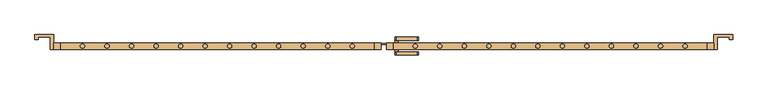
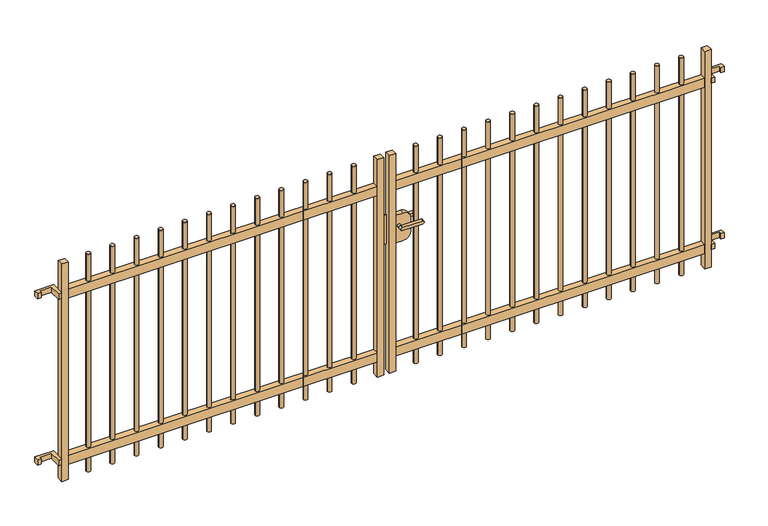
"""IFC4 building model written with IfcOpenShell, lengths in millimetres: door geometry, NLRS_90_DO_UN_draaipoort met spijlen 4000x1500_gen_rsf : draaipoort bxh 4000x1500mm-NP."""

import ifcopenshell
import ifcopenshell.guid

model = None  # the IFC model being written
_history = None  # IfcOwnerHistory: only IFC2X3 demands one
_inside = {}  # id of a spatial element -> (the spatial element, [elements in it])
_under = {}  # id of a project, library or spatial element -> (it, [spatial elements below it])
_declared = {}  # id of a project -> (the project, [libraries it declares])
_typed = {}  # id of a type object -> (the type object, [elements of that type])
_made_of = {}  # id of a material, layer set ... -> (it, [elements and type objects made of it])


def new_model(schema):
    """Start an empty IFC model of exactly this schema.

    Asked for "IFC4X3", IfcOpenShell would pick the latest addendum, in which some entities
    have other attributes; the version numbers below select the first issue.
    IFC2X3 requires an IfcOwnerHistory on every rooted entity: one is made here for all.
    """
    global model, _history
    if schema == "IFC4X3":
        model = ifcopenshell.file(schema_version=(4, 3, 0, 0))
    else:
        model = ifcopenshell.file(schema=schema)
    _inside.clear()
    _under.clear()
    _declared.clear()
    _typed.clear()
    _made_of.clear()
    _history = None
    if model.schema == "IFC2X3":
        org = make("IfcOrganization", Name="unknown")
        user = make(
            "IfcPersonAndOrganization",
            ThePerson=make("IfcPerson", FamilyName="unknown"),
            TheOrganization=org,
        )
        app = make(
            "IfcApplication",
            ApplicationDeveloper=org,
            Version="unknown",
            ApplicationFullName="unknown",
            ApplicationIdentifier="unknown",
        )
        _history = make(
            "IfcOwnerHistory",
            OwningUser=user,
            OwningApplication=app,
            ChangeAction="ADDED",
            CreationDate=0,
        )
    return model


def make(cls, **values):
    """One entity of the class cls with the attributes given. An attribute that is None is left unset."""
    return model.create_entity(
        cls, **{name: value for name, value in values.items() if value is not None}
    )


def rooted(cls, **values):
    """An entity with a GlobalId (a new one), such as an element, a storey or a relation."""
    return make(cls, GlobalId=ifcopenshell.guid.new(), OwnerHistory=_history, **values)


def si_unit(unit_type, name, prefix=None):
    """IfcSIUnit, for example si_unit("LENGTHUNIT", "METRE", prefix="MILLI")."""
    return make("IfcSIUnit", UnitType=unit_type, Prefix=prefix, Name=name)


def assignment(units):
    """IfcUnitAssignment: the units of a project."""
    return None if units is None else make("IfcUnitAssignment", Units=units)


def point(xyz):
    """IfcCartesianPoint."""
    return None if xyz is None else make("IfcCartesianPoint", Coordinates=xyz)


def direction(xyz):
    """IfcDirection."""
    return None if xyz is None else make("IfcDirection", DirectionRatios=xyz)


def frame(location, z_axis=None, x_axis=None):
    """IfcAxis2Placement3D, a coordinate frame: its origin and axes. An axis left out is left unset."""
    return make(
        "IfcAxis2Placement3D",
        Location=point(location),
        Axis=direction(z_axis),
        RefDirection=direction(x_axis),
    )


def frame_2d(location, x_axis=None):
    """IfcAxis2Placement2D, a coordinate frame in the plane: its origin and x axis."""
    return make(
        "IfcAxis2Placement2D", Location=point(location), RefDirection=direction(x_axis)
    )


def origin():
    """The frame at (0, 0, 0) with its axes left unset."""
    return frame((0.0, 0.0, 0.0))


def place(relative_to, where):
    """IfcLocalPlacement: puts the frame where relative to a parent placement (None: the world)."""
    return make(
        "IfcLocalPlacement", PlacementRelTo=relative_to, RelativePlacement=where
    )


def context(
    kind, dimensions, precision=None, world=None, true_north=None, identifier=None
):
    """IfcGeometricRepresentationContext, for example the 3D "Model" context."""
    return make(
        "IfcGeometricRepresentationContext",
        ContextIdentifier=identifier,
        ContextType=kind,
        CoordinateSpaceDimension=dimensions,
        Precision=precision,
        WorldCoordinateSystem=world,
        TrueNorth=true_north,
    )


def project(units=None, contexts=None):
    """IfcProject with its units and contexts."""
    return rooted(
        "IfcProject",
        Name="project",
        RepresentationContexts=contexts,
        UnitsInContext=assignment(units),
    )


def spatial(cls, under=None, at=None, **own):
    """A site, building, storey or space (cls), placed at a placement, below another one or the project."""
    s = rooted(cls, ObjectPlacement=at, **own)
    if under is not None:
        _under.setdefault(under.id(), (under, []))[1].append(s)
    return s


def polyline(points):
    """IfcPolyline through the points."""
    return make("IfcPolyline", Points=[point(p) for p in points])


def circle_curve(where, radius):
    """IfcCircle in the frame where."""
    return make("IfcCircle", Position=where, Radius=radius)


def trimmed(basis, trim1, trim2, sense, master):
    """IfcTrimmedCurve: the piece of a basis curve between two trims."""
    return make(
        "IfcTrimmedCurve",
        BasisCurve=basis,
        Trim1=trim1,
        Trim2=trim2,
        SenseAgreement=sense,
        MasterRepresentation=master,
    )


def segment(curve, same_sense, transition):
    """IfcCompositeCurveSegment."""
    return make(
        "IfcCompositeCurveSegment",
        Transition=transition,
        SameSense=same_sense,
        ParentCurve=curve,
    )


def composite_curve(segments, self_intersect=None):
    """IfcCompositeCurve: segments joined end to end."""
    return make("IfcCompositeCurve", Segments=segments, SelfIntersect=self_intersect)


def outline(outer, holes=None, kind="AREA"):
    """IfcArbitraryClosedProfileDef: a profile drawn as a closed curve; with holes, ...WithVoids."""
    if holes is None:
        return make("IfcArbitraryClosedProfileDef", ProfileType=kind, OuterCurve=outer)
    return make(
        "IfcArbitraryProfileDefWithVoids",
        ProfileType=kind,
        OuterCurve=outer,
        InnerCurves=holes,
    )


def extrude(swept, where, along, depth):
    """IfcExtrudedAreaSolid: the profile swept, set in the frame where, extruded along a direction by depth."""
    return make(
        "IfcExtrudedAreaSolid",
        SweptArea=swept,
        Position=where,
        ExtrudedDirection=direction(along),
        Depth=depth,
    )


def shape(context_of_items, identifier, shape_type, items):
    """IfcShapeRepresentation: the items that make up one representation, for example the "Body"."""
    return make(
        "IfcShapeRepresentation",
        ContextOfItems=context_of_items,
        RepresentationIdentifier=identifier,
        RepresentationType=shape_type,
        Items=items,
    )


def source(mapping_origin, context_of_items, identifier, shape_type, items):
    """IfcRepresentationMap: a shape defined once, which mapped items show again and again."""
    return make(
        "IfcRepresentationMap",
        MappingOrigin=mapping_origin,
        MappedRepresentation=shape(context_of_items, identifier, shape_type, items),
    )


def transform(
    local_origin,
    x_axis=None,
    y_axis=None,
    z_axis=None,
    scale=None,
    scale2=None,
    scale3=None,
    uniform=True,
):
    """IfcCartesianTransformationOperator3D, or its non-uniform kind. x_axis, y_axis, z_axis: its Axis1, 2, 3."""
    if uniform:
        return make(
            "IfcCartesianTransformationOperator3D",
            Axis1=direction(x_axis),
            Axis2=direction(y_axis),
            LocalOrigin=point(local_origin),
            Scale=scale,
            Axis3=direction(z_axis),
        )
    return make(
        "IfcCartesianTransformationOperator3DnonUniform",
        Axis1=direction(x_axis),
        Axis2=direction(y_axis),
        LocalOrigin=point(local_origin),
        Scale=scale,
        Axis3=direction(z_axis),
        Scale2=scale2,
        Scale3=scale3,
    )


def mapped(mapping_source, mapping_target):
    """IfcMappedItem: shows the shape of a source again, moved by a transform."""
    return make(
        "IfcMappedItem", MappingSource=mapping_source, MappingTarget=mapping_target
    )


def made_of(thing, what):
    """Note that an element or type object is made of a material, layer set ...; save() writes the relation."""
    if what is not None:
        _made_of.setdefault(what.id(), (what, []))[1].append(thing)
    return thing


def element(
    cls,
    number,
    at=None,
    inside=None,
    cuts=None,
    type_object=None,
    material=None,
    context=None,
    identifier="Body",
    shape_type=None,
    held_by="IfcProductDefinitionShape",
    body=None,
    shapes=None,
    **own,
):
    """One element of the class cls, such as IfcWall. Its Tag is "e" and its number.

    at: its placement. inside: the storey or other place that contains it. cuts: it is an
    opening in that element (IfcRelVoidsElement). A single representation is given by context,
    identifier, shape_type and body (its items); several are given by shapes. held_by: the class
    of the entity that holds the representations. save() writes the other relations.
    """
    e = rooted(cls, Tag="e%d" % number, ObjectPlacement=at, **own)
    if body is not None:
        shapes = [shape(context, identifier, shape_type, body)]
    if shapes is not None:
        e.Representation = make(held_by, Representations=shapes)
    if inside is not None:
        _inside.setdefault(inside.id(), (inside, []))[1].append(e)
    if cuts is not None:
        rooted(
            "IfcRelVoidsElement", RelatingBuildingElement=cuts, RelatedOpeningElement=e
        )
    if type_object is not None:
        _typed.setdefault(type_object.id(), (type_object, []))[1].append(e)
    return made_of(e, material)


def aggregate(whole, parts):
    """IfcRelAggregates: a whole, such as a stair, and the parts it consists of."""
    return rooted("IfcRelAggregates", RelatingObject=whole, RelatedObjects=parts)


def save(model, path):
    """Write the relations noted so far, then the file.

    IfcRelAggregates (storeys below a building ...), IfcRelContainedInSpatialStructure (elements
    in a storey), IfcRelDefinesByType, IfcRelAssociatesMaterial and IfcRelDeclares: one each for
    every whole, place, type object, material and project.
    """
    for whole, parts in _under.values():
        aggregate(whole, parts)
    for where, things in _inside.values():
        rooted(
            "IfcRelContainedInSpatialStructure",
            RelatedElements=things,
            RelatingStructure=where,
        )
    for kind, things in _typed.values():
        rooted("IfcRelDefinesByType", RelatedObjects=things, RelatingType=kind)
    for what, things in _made_of.values():
        rooted("IfcRelAssociatesMaterial", RelatedObjects=things, RelatingMaterial=what)
    for by, libraries in _declared.values():
        rooted("IfcRelDeclares", RelatingContext=by, RelatedDefinitions=libraries)
    model.write(path)


def door_459dbaae(model_context):
    return source(origin(), model_context, "Body", "SweptSolid", [
        extrude(outline(composite_curve([segment(trimmed(circle_curve(frame_2d((-1842.5, 0.0)), 13.0), [point((-1855.5, 1.1e-06))], [point((-1829.5, -1.1e-06))], False, "CARTESIAN"), True, "CONTINUOUS"), segment(trimmed(circle_curve(frame_2d((-1842.5, 0.0)), 13.0), [point((-1829.5, -1.1e-06))], [point((-1855.5, 1.1e-06))], False, "CARTESIAN"), True, "CONTINUOUS")], self_intersect=False)), frame((0.0, 0.0, 50.0), z_axis=(0.0, 0.0, 1.0), x_axis=(1.0, 0.0, 0.0)), (0.0, 0.0, 1.0), 1430.0),
        extrude(outline(composite_curve([segment(trimmed(circle_curve(frame_2d((-1692.5, 0.0)), 13.0), [point((-1705.5, 1.1e-06))], [point((-1679.5, -1.1e-06))], False, "CARTESIAN"), True, "CONTINUOUS"), segment(trimmed(circle_curve(frame_2d((-1692.5, 0.0)), 13.0), [point((-1679.5, -1.1e-06))], [point((-1705.5, 1.1e-06))], False, "CARTESIAN"), True, "CONTINUOUS")], self_intersect=False)), frame((0.0, 0.0, 50.0), z_axis=(0.0, 0.0, 1.0), x_axis=(1.0, 0.0, 0.0)), (0.0, 0.0, 1.0), 1430.0),
        extrude(outline(composite_curve([segment(trimmed(circle_curve(frame_2d((-1542.5, 0.0)), 13.0), [point((-1555.5, 1.1e-06))], [point((-1529.5, -1.1e-06))], False, "CARTESIAN"), True, "CONTINUOUS"), segment(trimmed(circle_curve(frame_2d((-1542.5, 0.0)), 13.0), [point((-1529.5, -1.1e-06))], [point((-1555.5, 1.1e-06))], False, "CARTESIAN"), True, "CONTINUOUS")], self_intersect=False)), frame((0.0, 0.0, 50.0), z_axis=(0.0, 0.0, 1.0), x_axis=(1.0, 0.0, 0.0)), (0.0, 0.0, 1.0), 1430.0),
        extrude(outline(composite_curve([segment(trimmed(circle_curve(frame_2d((-1392.5, 0.0)), 13.0), [point((-1405.5, 1.1e-06))], [point((-1379.5, -1.1e-06))], False, "CARTESIAN"), True, "CONTINUOUS"), segment(trimmed(circle_curve(frame_2d((-1392.5, 0.0)), 13.0), [point((-1379.5, -1.1e-06))], [point((-1405.5, 1.1e-06))], False, "CARTESIAN"), True, "CONTINUOUS")], self_intersect=False)), frame((0.0, 0.0, 50.0), z_axis=(0.0, 0.0, 1.0), x_axis=(1.0, 0.0, 0.0)), (0.0, 0.0, 1.0), 1430.0),
        extrude(outline(composite_curve([segment(trimmed(circle_curve(frame_2d((-1242.5, 0.0)), 13.0), [point((-1255.5, 1.1e-06))], [point((-1229.5, -1.1e-06))], False, "CARTESIAN"), True, "CONTINUOUS"), segment(trimmed(circle_curve(frame_2d((-1242.5, 0.0)), 13.0), [point((-1229.5, -1.1e-06))], [point((-1255.5, 1.1e-06))], False, "CARTESIAN"), True, "CONTINUOUS")], self_intersect=False)), frame((0.0, 0.0, 50.0), z_axis=(0.0, 0.0, 1.0), x_axis=(1.0, 0.0, 0.0)), (0.0, 0.0, 1.0), 1430.0),
        extrude(outline(composite_curve([segment(trimmed(circle_curve(frame_2d((-1092.5, 0.0)), 13.0), [point((-1105.5, 1.1e-06))], [point((-1079.5, -1.1e-06))], False, "CARTESIAN"), True, "CONTINUOUS"), segment(trimmed(circle_curve(frame_2d((-1092.5, 0.0)), 13.0), [point((-1079.5, -1.1e-06))], [point((-1105.5, 1.1e-06))], False, "CARTESIAN"), True, "CONTINUOUS")], self_intersect=False)), frame((0.0, 0.0, 50.0), z_axis=(0.0, 0.0, 1.0), x_axis=(1.0, 0.0, 0.0)), (0.0, 0.0, 1.0), 1430.0),
        extrude(outline(composite_curve([segment(trimmed(circle_curve(frame_2d((-942.5, 0.0)), 13.0), [point((-955.5, 1.1e-06))], [point((-929.5, -1.1e-06))], False, "CARTESIAN"), True, "CONTINUOUS"), segment(trimmed(circle_curve(frame_2d((-942.5, 0.0)), 13.0), [point((-929.5, -1.1e-06))], [point((-955.5, 1.1e-06))], False, "CARTESIAN"), True, "CONTINUOUS")], self_intersect=False)), frame((0.0, 0.0, 50.0), z_axis=(0.0, 0.0, 1.0), x_axis=(1.0, 0.0, 0.0)), (0.0, 0.0, 1.0), 1430.0),
        extrude(outline(composite_curve([segment(trimmed(circle_curve(frame_2d((-792.5, 0.0)), 13.0), [point((-805.5, 1.1e-06))], [point((-779.5, -1.1e-06))], False, "CARTESIAN"), True, "CONTINUOUS"), segment(trimmed(circle_curve(frame_2d((-792.5, 0.0)), 13.0), [point((-779.5, -1.1e-06))], [point((-805.5, 1.1e-06))], False, "CARTESIAN"), True, "CONTINUOUS")], self_intersect=False)), frame((0.0, 0.0, 50.0), z_axis=(0.0, 0.0, 1.0), x_axis=(1.0, 0.0, 0.0)), (0.0, 0.0, 1.0), 1430.0),
        extrude(outline(composite_curve([segment(trimmed(circle_curve(frame_2d((-642.5, 0.0)), 13.0), [point((-655.5, 1.1e-06))], [point((-629.5, -1.1e-06))], False, "CARTESIAN"), True, "CONTINUOUS"), segment(trimmed(circle_curve(frame_2d((-642.5, 0.0)), 13.0), [point((-629.5, -1.1e-06))], [point((-655.5, 1.1e-06))], False, "CARTESIAN"), True, "CONTINUOUS")], self_intersect=False)), frame((0.0, 0.0, 50.0), z_axis=(0.0, 0.0, 1.0), x_axis=(1.0, 0.0, 0.0)), (0.0, 0.0, 1.0), 1430.0),
        extrude(outline(composite_curve([segment(trimmed(circle_curve(frame_2d((-192.5, 0.0)), 13.0), [point((-205.5, 1.1e-06))], [point((-179.5, -1.1e-06))], False, "CARTESIAN"), True, "CONTINUOUS"), segment(trimmed(circle_curve(frame_2d((-192.5, 0.0)), 13.0), [point((-179.5, -1.1e-06))], [point((-205.5, 1.1e-06))], False, "CARTESIAN"), True, "CONTINUOUS")], self_intersect=False)), frame((0.0, 0.0, 50.0), z_axis=(0.0, 0.0, 1.0), x_axis=(1.0, 0.0, 0.0)), (0.0, 0.0, 1.0), 1430.0),
        extrude(outline(composite_curve([segment(trimmed(circle_curve(frame_2d((-342.5, 0.0)), 13.0), [point((-355.5, 1.1e-06))], [point((-329.5, -1.1e-06))], False, "CARTESIAN"), True, "CONTINUOUS"), segment(trimmed(circle_curve(frame_2d((-342.5, 0.0)), 13.0), [point((-329.5, -1.1e-06))], [point((-355.5, 1.1e-06))], False, "CARTESIAN"), True, "CONTINUOUS")], self_intersect=False)), frame((0.0, 0.0, 50.0), z_axis=(0.0, 0.0, 1.0), x_axis=(1.0, 0.0, 0.0)), (0.0, 0.0, 1.0), 1430.0),
        extrude(outline(composite_curve([segment(trimmed(circle_curve(frame_2d((-492.5, 0.0)), 13.0), [point((-505.5, 1.1e-06))], [point((-479.5, -1.1e-06))], False, "CARTESIAN"), True, "CONTINUOUS"), segment(trimmed(circle_curve(frame_2d((-492.5, 0.0)), 13.0), [point((-479.5, -1.1e-06))], [point((-505.5, 1.1e-06))], False, "CARTESIAN"), True, "CONTINUOUS")], self_intersect=False)), frame((0.0, 0.0, 50.0), z_axis=(0.0, 0.0, 1.0), x_axis=(1.0, 0.0, 0.0)), (0.0, 0.0, 1.0), 1430.0),
        extrude(outline(polyline([(-1977.5, -20.0), (-2017.5, -20.0), (-2017.5, 20.0), (-1977.5, 20.0), (-1977.5, -20.0)])), frame((0.0, 0.0, 50.0), z_axis=(0.0, 0.0, 1.0), x_axis=(1.0, 0.0, 0.0)), (0.0, 0.0, 1.0), 1430.0),
        extrude(outline(polyline([(-17.5, -20.0), (-57.5, -20.0), (-57.5, 20.0), (-17.5, 20.0), (-17.5, -20.0)])), frame((0.0, 0.0, 50.0), z_axis=(0.0, 0.0, 1.0), x_axis=(1.0, 0.0, 0.0)), (0.0, 0.0, 1.0), 1430.0),
        extrude(outline(composite_curve([segment(trimmed(circle_curve(frame_2d((1842.5, 0.0)), 13.0), [point((1855.5, 0.0))], [point((1829.5, 0.0))], False, "CARTESIAN"), True, "CONTINUOUS"), segment(trimmed(circle_curve(frame_2d((1842.5, 0.0)), 13.0), [point((1829.5, 0.0))], [point((1855.5, 0.0))], False, "CARTESIAN"), True, "CONTINUOUS")], self_intersect=False)), frame((0.0, 0.0, 50.0), z_axis=(0.0, 0.0, 1.0), x_axis=(1.0, 0.0, 0.0)), (0.0, 0.0, 1.0), 1430.0),
        extrude(outline(composite_curve([segment(trimmed(circle_curve(frame_2d((1692.5, 0.0)), 13.0), [point((1705.5, 0.0))], [point((1679.5, 0.0))], False, "CARTESIAN"), True, "CONTINUOUS"), segment(trimmed(circle_curve(frame_2d((1692.5, 0.0)), 13.0), [point((1679.5, 0.0))], [point((1705.5, 0.0))], False, "CARTESIAN"), True, "CONTINUOUS")], self_intersect=False)), frame((0.0, 0.0, 50.0), z_axis=(0.0, 0.0, 1.0), x_axis=(1.0, 0.0, 0.0)), (0.0, 0.0, 1.0), 1430.0),
        extrude(outline(composite_curve([segment(trimmed(circle_curve(frame_2d((1542.5, 0.0)), 13.0), [point((1555.5, 0.0))], [point((1529.5, 0.0))], False, "CARTESIAN"), True, "CONTINUOUS"), segment(trimmed(circle_curve(frame_2d((1542.5, 0.0)), 13.0), [point((1529.5, 0.0))], [point((1555.5, 0.0))], False, "CARTESIAN"), True, "CONTINUOUS")], self_intersect=False)), frame((0.0, 0.0, 50.0), z_axis=(0.0, 0.0, 1.0), x_axis=(1.0, 0.0, 0.0)), (0.0, 0.0, 1.0), 1430.0),
        extrude(outline(composite_curve([segment(trimmed(circle_curve(frame_2d((1392.5, 0.0)), 13.0), [point((1405.5, 0.0))], [point((1379.5, 0.0))], False, "CARTESIAN"), True, "CONTINUOUS"), segment(trimmed(circle_curve(frame_2d((1392.5, 0.0)), 13.0), [point((1379.5, 0.0))], [point((1405.5, 0.0))], False, "CARTESIAN"), True, "CONTINUOUS")], self_intersect=False)), frame((0.0, 0.0, 50.0), z_axis=(0.0, 0.0, 1.0), x_axis=(1.0, 0.0, 0.0)), (0.0, 0.0, 1.0), 1430.0),
        extrude(outline(composite_curve([segment(trimmed(circle_curve(frame_2d((1242.5, 0.0)), 13.0), [point((1255.5, 0.0))], [point((1229.5, 0.0))], False, "CARTESIAN"), True, "CONTINUOUS"), segment(trimmed(circle_curve(frame_2d((1242.5, 0.0)), 13.0), [point((1229.5, 0.0))], [point((1255.5, 0.0))], False, "CARTESIAN"), True, "CONTINUOUS")], self_intersect=False)), frame((0.0, 0.0, 50.0), z_axis=(0.0, 0.0, 1.0), x_axis=(1.0, 0.0, 0.0)), (0.0, 0.0, 1.0), 1430.0),
        extrude(outline(composite_curve([segment(trimmed(circle_curve(frame_2d((1092.5, 0.0)), 13.0), [point((1105.5, 0.0))], [point((1079.5, 0.0))], False, "CARTESIAN"), True, "CONTINUOUS"), segment(trimmed(circle_curve(frame_2d((1092.5, 0.0)), 13.0), [point((1079.5, 0.0))], [point((1105.5, 0.0))], False, "CARTESIAN"), True, "CONTINUOUS")], self_intersect=False)), frame((0.0, 0.0, 50.0), z_axis=(0.0, 0.0, 1.0), x_axis=(1.0, 0.0, 0.0)), (0.0, 0.0, 1.0), 1430.0),
        extrude(outline(composite_curve([segment(trimmed(circle_curve(frame_2d((942.5, 0.0)), 13.0), [point((955.5, 0.0))], [point((929.5, 0.0))], False, "CARTESIAN"), True, "CONTINUOUS"), segment(trimmed(circle_curve(frame_2d((942.5, 0.0)), 13.0), [point((929.5, 0.0))], [point((955.5, 0.0))], False, "CARTESIAN"), True, "CONTINUOUS")], self_intersect=False)), frame((0.0, 0.0, 50.0), z_axis=(0.0, 0.0, 1.0), x_axis=(1.0, 0.0, 0.0)), (0.0, 0.0, 1.0), 1430.0),
        extrude(outline(composite_curve([segment(trimmed(circle_curve(frame_2d((792.5, 0.0)), 13.0), [point((805.5, 0.0))], [point((779.5, 0.0))], False, "CARTESIAN"), True, "CONTINUOUS"), segment(trimmed(circle_curve(frame_2d((792.5, 0.0)), 13.0), [point((779.5, 0.0))], [point((805.5, 0.0))], False, "CARTESIAN"), True, "CONTINUOUS")], self_intersect=False)), frame((0.0, 0.0, 50.0), z_axis=(0.0, 0.0, 1.0), x_axis=(1.0, 0.0, 0.0)), (0.0, 0.0, 1.0), 1430.0),
        extrude(outline(composite_curve([segment(trimmed(circle_curve(frame_2d((642.5, 0.0)), 13.0), [point((655.5, 0.0))], [point((629.5, 0.0))], False, "CARTESIAN"), True, "CONTINUOUS"), segment(trimmed(circle_curve(frame_2d((642.5, 0.0)), 13.0), [point((629.5, 0.0))], [point((655.5, 0.0))], False, "CARTESIAN"), True, "CONTINUOUS")], self_intersect=False)), frame((0.0, 0.0, 50.0), z_axis=(0.0, 0.0, 1.0), x_axis=(1.0, 0.0, 0.0)), (0.0, 0.0, 1.0), 1430.0),
        extrude(outline(composite_curve([segment(trimmed(circle_curve(frame_2d((192.5, 0.0)), 13.0), [point((205.5, 0.0))], [point((179.5, 0.0))], False, "CARTESIAN"), True, "CONTINUOUS"), segment(trimmed(circle_curve(frame_2d((192.5, 0.0)), 13.0), [point((179.5, 0.0))], [point((205.5, 0.0))], False, "CARTESIAN"), True, "CONTINUOUS")], self_intersect=False)), frame((0.0, 0.0, 50.0), z_axis=(0.0, 0.0, 1.0), x_axis=(1.0, 0.0, 0.0)), (0.0, 0.0, 1.0), 1430.0),
        extrude(outline(composite_curve([segment(trimmed(circle_curve(frame_2d((342.5, 0.0)), 13.0), [point((355.5, 0.0))], [point((329.5, 0.0))], False, "CARTESIAN"), True, "CONTINUOUS"), segment(trimmed(circle_curve(frame_2d((342.5, 0.0)), 13.0), [point((329.5, 0.0))], [point((355.5, 0.0))], False, "CARTESIAN"), True, "CONTINUOUS")], self_intersect=False)), frame((0.0, 0.0, 50.0), z_axis=(0.0, 0.0, 1.0), x_axis=(1.0, 0.0, 0.0)), (0.0, 0.0, 1.0), 1430.0),
        extrude(outline(composite_curve([segment(trimmed(circle_curve(frame_2d((492.5, 0.0)), 13.0), [point((505.5, 0.0))], [point((479.5, 0.0))], False, "CARTESIAN"), True, "CONTINUOUS"), segment(trimmed(circle_curve(frame_2d((492.5, 0.0)), 13.0), [point((479.5, 0.0))], [point((505.5, 0.0))], False, "CARTESIAN"), True, "CONTINUOUS")], self_intersect=False)), frame((0.0, 0.0, 50.0), z_axis=(0.0, 0.0, 1.0), x_axis=(1.0, 0.0, 0.0)), (0.0, 0.0, 1.0), 1430.0),
        extrude(outline(polyline([(1977.5, -20.0), (1977.5, 20.0), (2017.5, 20.0), (2017.5, -20.0), (1977.5, -20.0)])), frame((0.0, 0.0, 50.0), z_axis=(0.0, 0.0, 1.0), x_axis=(1.0, 0.0, 0.0)), (0.0, 0.0, 1.0), 1430.0),
        extrude(outline(polyline([(17.5, -20.0), (17.5, 20.0), (57.5, 20.0), (57.5, -20.0), (17.5, -20.0)])), frame((0.0, 0.0, 50.0), z_axis=(0.0, 0.0, 1.0), x_axis=(1.0, 0.0, 0.0)), (0.0, 0.0, 1.0), 1430.0),
        extrude(outline(composite_curve([segment(polyline([(1008.625, 203.3906246), (1008.625, 78.3906258)]), True, "CONTINUOUS"), segment(trimmed(circle_curve(frame_2d((998.625, 78.390625)), 10.0), [point((1008.625, 78.3906258))], [point((988.625, 78.390625))], False, "CARTESIAN"), True, "CONTINUOUS"), segment(polyline([(988.625, 78.390625), (988.625, 203.3906269)]), True, "CONTINUOUS"), segment(trimmed(circle_curve(frame_2d((998.625, 203.390625)), 10.0), [point((988.625, 203.3906269))], [point((1008.625, 203.3906246))], False, "CARTESIAN"), True, "CONTINUOUS")], self_intersect=False)), frame((0.0, 35.0, 0.0), z_axis=(0.0, 1.0, 0.0), x_axis=(0.0, 0.0, 1.0)), (0.0, 0.0, 1.0), 20.0),
        extrude(outline(composite_curve([segment(polyline([(1008.625, 203.3906246), (1008.625, 78.3906258)]), True, "CONTINUOUS"), segment(trimmed(circle_curve(frame_2d((998.625, 78.390625)), 10.0), [point((1008.625, 78.3906258))], [point((988.625, 78.390625))], False, "CARTESIAN"), True, "CONTINUOUS"), segment(polyline([(988.625, 78.390625), (988.625, 203.3906269)]), True, "CONTINUOUS"), segment(trimmed(circle_curve(frame_2d((998.625, 203.390625)), 10.0), [point((988.625, 203.3906269))], [point((1008.625, 203.3906246))], False, "CARTESIAN"), True, "CONTINUOUS")], self_intersect=False)), frame((0.0, -55.0, 0.0), z_axis=(0.0, 1.0, 0.0), x_axis=(0.0, 0.0, 1.0)), (0.0, 0.0, 1.0), 20.0),
        extrude(outline(polyline([(37.5, 10.0), (-17.5, 10.0), (-17.5, 15.0), (37.5, 15.0), (37.5, 10.0)])), frame((0.0, 0.0, 885.0625), z_axis=(0.0, 0.0, 1.0), x_axis=(1.0, 0.0, 0.0)), (0.0, 0.0, 1.0), 190.0),
        extrude(outline(composite_curve([segment(polyline([(1070.0, 57.5), (890.0, 57.5), (890.0, 107.499998)]), True, "CONTINUOUS"), segment(trimmed(circle_curve(frame_2d((935.0, 107.5)), 45.0), [point((890.0, 107.499998))], [point((935.0, 152.5))], False, "CARTESIAN"), True, "CONTINUOUS"), segment(polyline([(935.0, 152.5), (1025.0, 152.5)]), True, "CONTINUOUS"), segment(trimmed(circle_curve(frame_2d((1025.0, 107.5)), 45.0), [point((1025.0, 152.5))], [point((1070.0, 107.5))], False, "CARTESIAN"), True, "CONTINUOUS"), segment(polyline([(1070.0, 107.5), (1070.0, 57.5)]), True, "CONTINUOUS")], self_intersect=False)), frame((0.0, -15.0, 0.0), z_axis=(0.0, 1.0, 0.0), x_axis=(0.0, 0.0, 1.0)), (0.0, 0.0, 1.0), 30.0),
        extrude(outline(composite_curve([segment(trimmed(circle_curve(frame_2d((998.625, 78.390625)), 10.0), [point((998.6250009, 68.390625))], [point((998.6249991, 88.390625))], False, "CARTESIAN"), True, "CONTINUOUS"), segment(trimmed(circle_curve(frame_2d((998.625, 78.390625)), 10.0), [point((998.6249991, 88.390625))], [point((998.6250009, 68.390625))], False, "CARTESIAN"), True, "CONTINUOUS")], self_intersect=False)), frame((0.0, 15.0, 0.0), z_axis=(0.0, 1.0, 0.0), x_axis=(0.0, 0.0, 1.0)), (0.0, 0.0, 1.0), 20.0),
        extrude(outline(composite_curve([segment(trimmed(circle_curve(frame_2d((998.625, 78.390625)), 10.0), [point((998.6250009, 68.390625))], [point((998.6249991, 88.390625))], False, "CARTESIAN"), True, "CONTINUOUS"), segment(trimmed(circle_curve(frame_2d((998.625, 78.390625)), 10.0), [point((998.6249991, 88.390625))], [point((998.6250009, 68.390625))], False, "CARTESIAN"), True, "CONTINUOUS")], self_intersect=False)), frame((0.0, -35.0, 0.0), z_axis=(0.0, 1.0, 0.0), x_axis=(0.0, 0.0, 1.0)), (0.0, 0.0, 1.0), 20.0),
        extrude(outline(polyline([(-2017.5, -20.0), (-2038.5, -20.0), (-2038.5, 56.65625), (-2112.25, 56.65625), (-2112.25, 40.0), (-2133.5, 40.0), (-2133.5, 70.0), (-2017.5, 70.0), (-2017.5, -20.0)])), frame((0.0, 0.0, 1256.1498273), z_axis=(0.0, 0.0, 1.0), x_axis=(1.0, 0.0, 0.0)), (0.0, 0.0, 1.0), 35.0),
        extrude(outline(polyline([(-57.5, -20.0), (-1977.5, -20.0), (-1977.5, 20.0), (-57.5, 20.0), (-57.5, -20.0)])), frame((0.0, 0.0, 1243.6498273), z_axis=(0.0, 0.0, 1.0), x_axis=(1.0, 0.0, 0.0)), (0.0, 0.0, 1.0), 60.0),
        extrude(outline(polyline([(-2017.5, -20.0), (-2038.5, -20.0), (-2038.5, 56.65625), (-2112.25, 56.65625), (-2112.25, 40.0), (-2133.5, 40.0), (-2133.5, 70.0), (-2017.5, 70.0), (-2017.5, -20.0)])), frame((0.0, 0.0, 162.5), z_axis=(0.0, 0.0, 1.0), x_axis=(1.0, 0.0, 0.0)), (0.0, 0.0, 1.0), 35.0),
        extrude(outline(polyline([(-57.5, -20.0), (-1977.5, -20.0), (-1977.5, 20.0), (-57.5, 20.0), (-57.5, -20.0)])), frame((0.0, 0.0, 150.0), z_axis=(0.0, 0.0, 1.0), x_axis=(1.0, 0.0, 0.0)), (0.0, 0.0, 1.0), 60.0),
        extrude(outline(polyline([(2017.5, -20.0), (2017.5, 70.0), (2133.5, 70.0), (2133.5, 40.0), (2112.25, 40.0), (2112.25, 56.65625), (2038.5, 56.65625), (2038.5, -20.0), (2017.5, -20.0)])), frame((0.0, 0.0, 1256.1498273), z_axis=(0.0, 0.0, 1.0), x_axis=(1.0, 0.0, 0.0)), (0.0, 0.0, 1.0), 35.0),
        extrude(outline(polyline([(57.5, -20.0), (57.5, 20.0), (1977.5, 20.0), (1977.5, -20.0), (57.5, -20.0)])), frame((0.0, 0.0, 1243.6498273), z_axis=(0.0, 0.0, 1.0), x_axis=(1.0, 0.0, 0.0)), (0.0, 0.0, 1.0), 60.0),
        extrude(outline(polyline([(2017.5, -20.0), (2017.5, 70.0), (2133.5, 70.0), (2133.5, 40.0), (2112.25, 40.0), (2112.25, 56.65625), (2038.5, 56.65625), (2038.5, -20.0), (2017.5, -20.0)])), frame((0.0, 0.0, 162.5), z_axis=(0.0, 0.0, 1.0), x_axis=(1.0, 0.0, 0.0)), (0.0, 0.0, 1.0), 35.0),
        extrude(outline(polyline([(57.5, -20.0), (57.5, 20.0), (1977.5, 20.0), (1977.5, -20.0), (57.5, -20.0)])), frame((0.0, 0.0, 150.0), z_axis=(0.0, 0.0, 1.0), x_axis=(1.0, 0.0, 0.0)), (0.0, 0.0, 1.0), 60.0),
    ])


if __name__ == "__main__":
    model = new_model("IFC4")
    model_context = context("Model", 3, world=origin())
    ifc_project = project(units=[si_unit("LENGTHUNIT", "METRE", prefix="MILLI")], contexts=[model_context])
    site = spatial("IfcSite", under=ifc_project)
    building = spatial("IfcBuilding", under=site)
    placement = place(None, origin())
    door_shape = door_459dbaae(model_context)
    element("IfcDoor", 1, ObjectType="NLRS_90_DO_UN_draaipoort met spijlen 4000x1500_gen_rsf : draaipoort bxh 4000x1500mm-NP", at=placement, inside=building, context=model_context, shape_type="MappedRepresentation", body=[
        mapped(door_shape, transform((0.0, 0.0, 0.0), x_axis=(1.0, 0.0, 0.0), y_axis=(0.0, 1.0, 0.0), z_axis=(0.0, 0.0, 1.0))),
    ])
    save(model, "model.ifc")

# Revit data of these elements
# Type "NLRS_90_DO_UN_draaipoort met spijlen 4000x1500_gen_rsf : draaipoort bxh 4000x1500mm-NP"
#   Type IFC Predefined Type = "GATE"
#   Export Type to IFC As = "IfcDoorType"
#   Type IfcGUID = "1A81voHkv98RYujw6ZYnw6"
#   IfcName[Type] = "draaipoort bxh 4000x1500mm-NP"
#   IfcDescription[Type] = "toegangspoort stalen spijlen bxh 4000x1500mm"
#   IfcExportAs[Type] = "IfcDoorType"
#   IfcExportType[Type] = "GATE"
#   NLRS_C_revit_versie = ""
#   NLRS_C_omschrijving_03 [instance default] = "doorgangsmaat"
#   NLRS_C_omschrijving_02 [instance default] = "sluiting"
#   NLRS_C_omschrijving_01 [instance default] = "poort"
#   NLRS_C_content_versie = ""
#   NLRS_C_content_provider = ""
#   NLRS_C_content_handleiding = ""
#   NLRS_C_content_datum_uitgifte = ""
#   NLRS_C_content_datum_gewijzigd = ""
#   NLRS_C_content_creator = ""
#   Model = "generiek"
#   Manufacturer = "Revit Standards Foundation"
#   Description = "toegangspoort stalen spijlen bxh 4000x1500mm"
#   Assembly Code = "90.32"
#   NLRS_C_hoogte = 1500.00 mm
#   NLRS_C_breedte_03 = 4130.00 mm
#   NLRS_C_breedte = 4165.00 mm
#   kolom rechts = no
#   kolom links = no
#   NLRS_C_materiaal_02 = NLRS_h_metaal_gen_rsf
#   NLRS_C_materiaal_01 = NLRS_h2_staal blauwgrijs_gen_rsf
#   URL = ""
#   Keynote = ""
#   Default Elevation = 0
# Element 1 (IfcDoor, "NLRS_90_DO_UN_draaipoort met spijlen 4000x1500_gen_rsf : draaipoort bxh 4000x1500mm-NP")
#   Materials on its faces: "NLRS_h2_staal blauwgrijs_gen_rsf", "NLRS_h_metaal_gen_rsf"
# Materials
#   "NLRS_h_metaal_gen_rsf": class "BCB class", colour RGB 149 148 153, transparency 0, Keynote = "h", Model = "generiek", Manufacturer = "Revit Standards Foundation", URL = "www.revitstandards.org", Description = "metaal", Cost = 0
#   "NLRS_h2_staal blauwgrijs_gen_rsf": class "BCB class", colour RGB 113 134 165, transparency 0, Keynote = "h2", Model = "generiek", Manufacturer = "Revit Standards Foundation", URL = "www.revitstandards.org", Description = "staal blauwgrijs", Cost = 0
